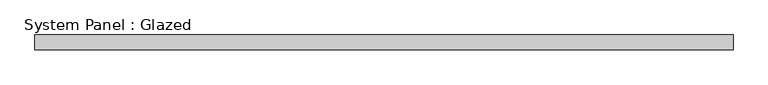
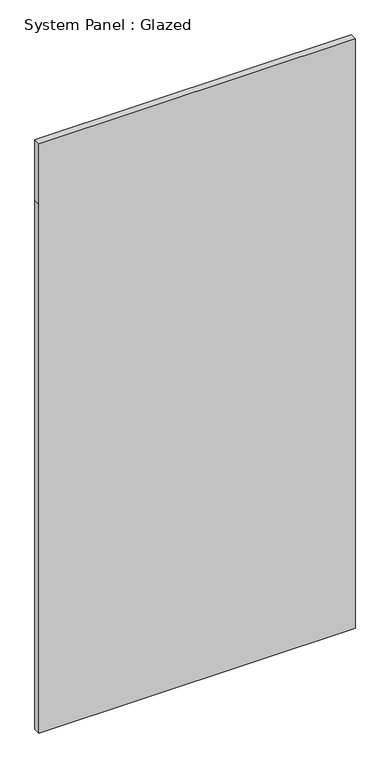
"""IFC4 building model written with IfcOpenShell, lengths in millimetres: plate geometry, System Panel : Glazed."""

from ifc_helpers import new_model, si_unit, frame, origin, place, context, project, spatial, polyline, outline, extrude, source, transform, mapped, element, save


def system_panel_glazed_1b64d018(model_context):
    return source(origin(), model_context, "Body", "SweptSolid", [
        extrude(outline(polyline([(0.0, -594.4075643), (0.0, 594.4075643), (2101.85, 594.4075643), (2343.15, 594.4075643), (2343.15, -594.4075643), (2101.85, -594.4075643), (0.0, -594.4075643)])), frame((0.0, 19.05, 0.0), z_axis=(0.0, 1.0, 0.0), x_axis=(0.0, 0.0, 1.0)), (0.0, 0.0, 1.0), 25.4),
    ])


if __name__ == "__main__":
    model = new_model("IFC4")
    model_context = context("Model", 3, world=origin())
    ifc_project = project(units=[si_unit("LENGTHUNIT", "METRE", prefix="MILLI")], contexts=[model_context])
    site = spatial("IfcSite", under=ifc_project)
    building = spatial("IfcBuilding", under=site)
    placement = place(None, origin())
    system_panel_glazed_shape = system_panel_glazed_1b64d018(model_context)
    element("IfcPlate", 1, ObjectType="System Panel : Glazed", at=placement, inside=building, context=model_context, shape_type="MappedRepresentation", body=[
        mapped(system_panel_glazed_shape, transform((0.0, 0.0, 0.0), x_axis=(1.0, 0.0, 0.0), y_axis=(0.0, 1.0, 0.0), z_axis=(0.0, 0.0, 1.0))),
    ])
    save(model, "model.ifc")

# Revit data of these elements
# Element 1 (IfcPlate, "System Panel : Glazed")
#   Materials on its faces: "Glass"
# Materials
#   "Glass": class "Glass", colour RGB 0 128 192, transparency 0.75
